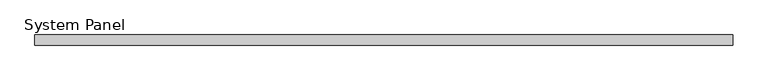
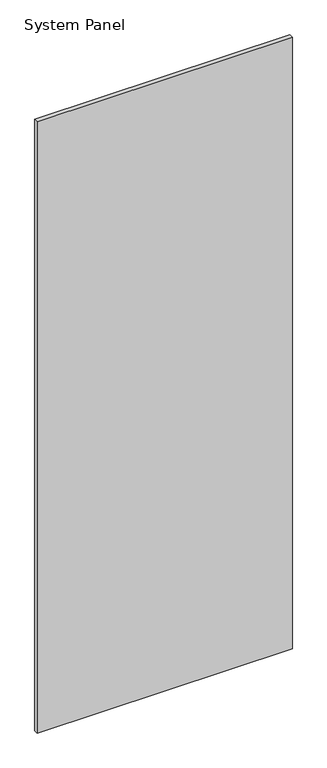
"""IFC4 building model written with IfcOpenShell, lengths in millimetres: plate geometry, System Panel : WWm-Glass-20mm-10mmOffset."""

from ifc_helpers import new_model, si_unit, origin, origin_with_axes, place, context, project, spatial, polyline, outline, extrude, source, transform, mapped, element, save


def system_panel_3ee36236(model_context):
    return source(origin(), model_context, "Body", "SweptSolid", [
        extrude(outline(polyline([(661.801525, 0.0), (-661.801525, 0.0), (-661.801525, 20.0), (661.801525, 20.0), (661.801525, 0.0)])), origin_with_axes(), (0.0, 0.0, 1.0), 3350.0),
    ])


if __name__ == "__main__":
    model = new_model("IFC4")
    model_context = context("Model", 3, world=origin())
    ifc_project = project(units=[si_unit("LENGTHUNIT", "METRE", prefix="MILLI")], contexts=[model_context])
    site = spatial("IfcSite", under=ifc_project)
    building = spatial("IfcBuilding", under=site)
    placement = place(None, origin())
    system_panel_shape = system_panel_3ee36236(model_context)
    element("IfcPlate", 1, ObjectType="System Panel : WWm-Glass-20mm-10mmOffset", at=placement, inside=building, context=model_context, shape_type="MappedRepresentation", body=[
        mapped(system_panel_shape, transform((0.0, 0.0, 0.0), x_axis=(1.0, 0.0, 0.0), y_axis=(0.0, 1.0, 0.0), z_axis=(0.0, 0.0, 1.0))),
    ])
    save(model, "model.ifc")

# Revit data of these elements
# Type "System Panel : WWm-Glass-20mm-10mmOffset"
#   Finish = ""
# Element 1 (IfcPlate, "System Panel : WWm-Glass-20mm-10mmOffset")
#   Materials on its faces: "WW-EC-GL-Storefront"
# Materials
#   "WW-EC-GL-Storefront": class "Glass", colour RGB 236 240 239, transparency 0.85, Description = "Storefront Glass", Cost = 0
